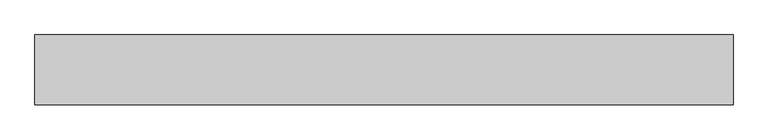
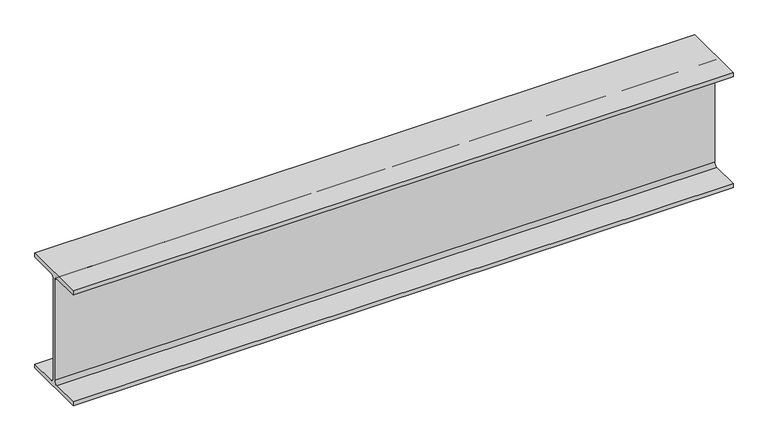
"""IFC4 building model written with IfcOpenShell, lengths in millimetres: beam geometry, Steel Beam_H-KSD3502 : H_SB_ASB_H-194x150x6x9."""

from ifc_helpers import new_model, si_unit, point, frame, frame_2d, origin, place, context, project, spatial, polyline, circle_curve, trimmed, segment, composite_curve, outline, extrude, source, transform, mapped, element, save


def beam_24535466(model_context):
    return source(origin(), model_context, "Body", "SweptSolid", [
        extrude(outline(composite_curve([segment(polyline([(-82.5, -141.5), (-11.9, -141.5)]), True, "CONTINUOUS"), segment(trimmed(circle_curve(frame_2d((-11.9, -132.6)), 8.9), [point((-11.9, -141.5))], [point((-3.0, -132.6))], True, "CARTESIAN"), True, "CONTINUOUS"), segment(polyline([(-3.0, -132.6), (-3.0, 132.6)]), True, "CONTINUOUS"), segment(trimmed(circle_curve(frame_2d((-11.9, 132.6)), 8.9), [point((-3.0, 132.6))], [point((-11.9, 141.5))], True, "CARTESIAN"), True, "CONTINUOUS"), segment(polyline([(-11.9, 141.5), (-82.5, 141.5), (-82.5, 151.7), (82.5, 151.7), (82.5, 141.5), (11.9, 141.5)]), True, "CONTINUOUS"), segment(trimmed(circle_curve(frame_2d((11.9, 132.6)), 8.9), [point((11.9, 141.5))], [point((3.0, 132.6))], True, "CARTESIAN"), True, "CONTINUOUS"), segment(polyline([(3.0, 132.6), (3.0, -132.6)]), True, "CONTINUOUS"), segment(trimmed(circle_curve(frame_2d((11.9, -132.6)), 8.9), [point((3.0, -132.6))], [point((11.9, -141.5))], True, "CARTESIAN"), True, "CONTINUOUS"), segment(polyline([(11.9, -141.5), (82.5, -141.5), (82.5, -151.7), (-82.5, -151.7), (-82.5, -141.5)]), True, "CONTINUOUS")], self_intersect=False)), frame((-700.4863388, 0.0, 0.0), z_axis=(1.0, 0.0, 0.0), x_axis=(0.0, 1.0, 0.0)), (0.0, 0.0, 1.0), 1647.7868301),
    ])


if __name__ == "__main__":
    model = new_model("IFC4")
    model_context = context("Model", 3, world=origin())
    ifc_project = project(units=[si_unit("LENGTHUNIT", "METRE", prefix="MILLI")], contexts=[model_context])
    site = spatial("IfcSite", under=ifc_project)
    building = spatial("IfcBuilding", under=site)
    placement = place(None, origin())
    beam_shape = beam_24535466(model_context)
    element("IfcBeam", 1, ObjectType="Steel Beam_H-KSD3502 : H_SB_ASB_H-194x150x6x9", at=placement, inside=building, context=model_context, shape_type="MappedRepresentation", body=[
        mapped(beam_shape, transform((0.0, 0.0, 0.0), x_axis=(1.0, 0.0, 0.0), y_axis=(0.0, 1.0, 0.0), z_axis=(0.0, 0.0, 1.0))),
    ])
    save(model, "model.ifc")

# Revit data of these elements
# Type "Steel Beam_H-KSD3502 : H_SB_ASB_H-194x150x6x9"
#   Width = 15.0 cm
#   Web Thickness = 0.6 cm
#   Web Fillet = 1.3 cm
#   Warping Constant = 43316.0 cm⁶
#   Torsional Moment of Inertia = 8.622 cm⁴
#   Torsional Modulus = 1.0 cm³
#   Section Area = 39.01 cm²
#   Plastic Modulus weak axis = 104.0 cm³
#   Plastic Modulus strong axis = 309.0 cm³
#   Perimeter = 0.95 m²/m
#   Nominal Weight = 30.60 kgf/m
#   Moment of Inertia weak axis = 507.00 cm⁴
#   Moment of Inertia strong axis = 2690.00 cm⁴
#   Height = 19.4 cm
#   Flange Thickness = 0.9 cm
#   Elastic Modulus weak axis = 67.6 cm³
#   Elastic Modulus strong axis = 277.0 cm³
#   Centroid Vertical = 9.7 cm
#   Centroid Horizontal = 7.5 cm
#   Length [instance default] = 1.5240 m
#   Structural Material [instance default] = Steel, 45-345
#   Assembly Code = ""
# Element 1 (IfcBeam, "Steel Beam_H-KSD3502 : H_SB_ASB_H-194x150x6x9")
#   Structural Material = none
# Materials
#   "Steel, 45-345": class "Metal", colour RGB 189 187 185, transparency 0, Description = "Steel 345 MPa", Cost = 0
